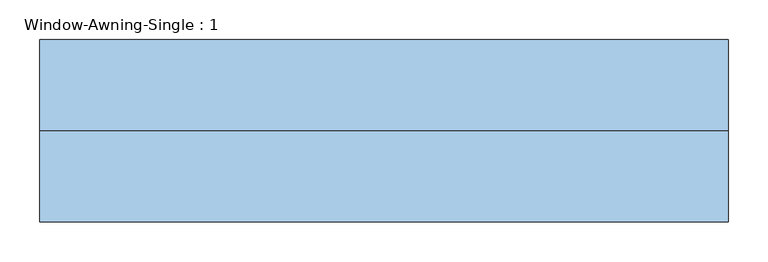
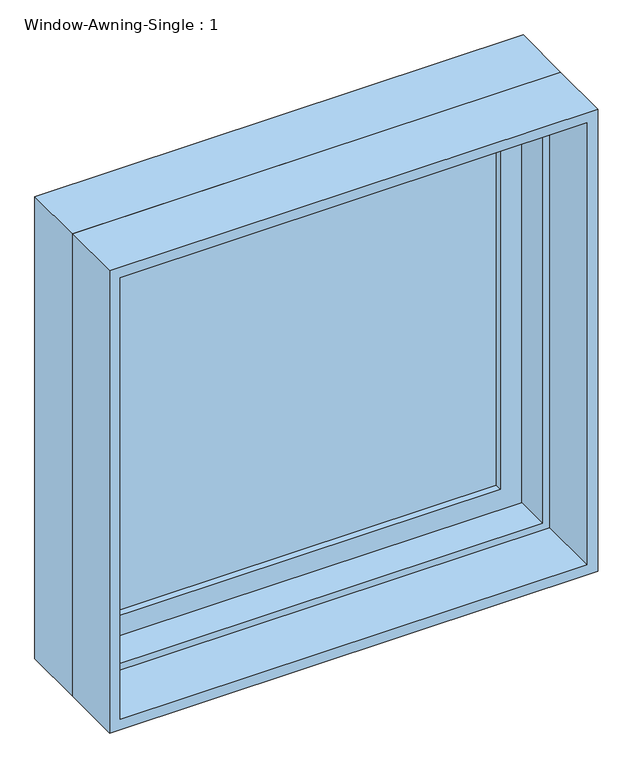
"""IFC4 building model written with IfcOpenShell, lengths in millimetres: window geometry, Window-Awning-Single : 1."""

from ifc_helpers import new_model, si_unit, frame, origin, place, context, project, spatial, polyline, outline, extrude, faceted_brep, source, transform, mapped, element, save


def window_awning_single_1_f21cafb6(model_context):
    return source(origin(), model_context, "Body", "SolidModel", [
        faceted_brep([(419.1, 73.025, 927.1), (419.1, 123.825, 927.1), (-419.1, 123.825, 927.1), (-419.1, 73.025, 927.1), (400.05, 9.525, 946.15), (400.05, 73.025, 946.15), (-400.05, 73.025, 946.15), (-400.05, 9.525, 946.15), (431.8, 123.825, 914.4), (431.8, 9.525, 914.4), (-431.8, 9.525, 914.4), (-431.8, 123.825, 914.4), (-419.1, 123.825, 1765.3), (-419.1, 73.025, 1765.3), (-400.05, 73.025, 1746.25), (-400.05, 9.525, 1746.25), (-431.8, 9.525, 1778.0), (-431.8, 123.825, 1778.0), (419.1, 123.825, 1765.3), (419.1, 73.025, 1765.3), (400.05, 73.025, 1746.25), (400.05, 9.525, 1746.25), (431.8, 9.525, 1778.0), (431.8, 123.825, 1778.0)], [[[0, 1, 2, 3]], [[4, 5, 6, 7]], [[8, 9, 10, 11]], [[3, 2, 12, 13]], [[7, 6, 14, 15]], [[11, 10, 16, 17]], [[13, 12, 18, 19]], [[15, 14, 20, 21]], [[17, 16, 22, 23]], [[11, 17, 23, 8], [1, 18, 12, 2]], [[19, 18, 1, 0]], [[3, 13, 19, 0], [5, 20, 14, 6]], [[21, 20, 5, 4]], [[9, 22, 16, 10], [7, 15, 21, 4]], [[23, 22, 9, 8]]]),
        extrude(outline(polyline([(361.95, 104.775), (361.95, 98.425), (-361.95, 98.425), (-361.95, 104.775), (361.95, 104.775)])), frame((0.0, 0.0, 984.25), z_axis=(0.0, 0.0, 1.0), x_axis=(1.0, 0.0, 0.0)), (0.0, 0.0, 1.0), 723.9),
        extrude(outline(polyline([(361.95, 92.075), (361.95, 85.725), (-361.95, 85.725), (-361.95, 92.075), (361.95, 92.075)])), frame((0.0, 0.0, 984.25), z_axis=(0.0, 0.0, 1.0), x_axis=(1.0, 0.0, 0.0)), (0.0, 0.0, 1.0), 723.9),
        extrude(outline(polyline([(927.1, -419.1), (927.1, 419.1), (1765.3, 419.1), (1765.3, -419.1), (927.1, -419.1)]), holes=[polyline([(1708.15, -361.95), (1708.15, 361.95), (984.25, 361.95), (984.25, -361.95), (1708.15, -361.95)])]), frame((0.0, 73.025, 0.0), z_axis=(0.0, 1.0, 0.0), x_axis=(0.0, 0.0, 1.0)), (0.0, 0.0, 1.0), 44.45),
        extrude(outline(polyline([(1778.0, -431.8), (914.4, -431.8), (914.4, 431.8), (1778.0, 431.8), (1778.0, -431.8)]), holes=[polyline([(1758.95, -412.75), (1758.95, 412.75), (933.45, 412.75), (933.45, -412.75), (1758.95, -412.75)])]), frame((0.0, -104.775, 0.0), z_axis=(0.0, 1.0, 0.0), x_axis=(0.0, 0.0, 1.0)), (0.0, 0.0, 1.0), 114.3),
    ])


if __name__ == "__main__":
    model = new_model("IFC4")
    model_context = context("Model", 3, world=origin())
    ifc_project = project(units=[si_unit("LENGTHUNIT", "METRE", prefix="MILLI")], contexts=[model_context])
    site = spatial("IfcSite", under=ifc_project)
    building = spatial("IfcBuilding", under=site)
    placement = place(None, origin())
    window_awning_single_1_shape = window_awning_single_1_f21cafb6(model_context)
    element("IfcWindow", 1, ObjectType="Window-Awning-Single : 1", at=placement, inside=building, context=model_context, shape_type="MappedRepresentation", body=[
        mapped(window_awning_single_1_shape, transform((0.0, 0.0, 0.0), x_axis=(1.0, 0.0, 0.0), y_axis=(0.0, 1.0, 0.0), z_axis=(0.0, 0.0, 1.0))),
    ])
    save(model, "model.ifc")

# Revit data of these elements
# Type "Window-Awning-Single : 1"
#   Type Mark = "14"
#   Fire Rating = "0.5h"
#   Assembly Code = "B2020100"
#   Analytic Construction = "Double glazing - domestic"
#   Window Inset [instance default] = 0' - 0"
#   Wall Thickness [instance default] = 0' - 6"
#   Visual Light Transmittance = 0.81
#   Thermal Resistance (R) = 0.319569 (m²·K)/W
#   Solar Heat Gain Coefficient = 0.76
#   Rough Width = 2' - 10 1/2"
#   Rough Height = 2' - 10 1/2"
#   Interior Wall Closure [instance default] = 0' - 2 1/4"
#   Height = 2' - 10"
#   Heat Transfer Coefficient (U) = 3.12929 W/(m²·K)
#   Frame Extension [instance default] = 0' - 0 1/4"
#   Exterior Wall Closure [instance default] = 0' - 1 1/4"
#   Extension Jamb [instance default] = 0' - 2 1/4"
#   Default Sill Height = 3' - 0"
#   Width = 2' - 10"
#   Muntin Visibility = yes
#   Interior Trim Visibility [instance default] = yes
#   Exterior Trim Visibility [instance default] = yes
#   Extension Jamb Visibility [instance default] = yes
#   Muntin Pattern = Muntin Pattern_2x2 : Muntin Pattern_2x2
#   Interior Trim Material = 1X WOOD COMPOSITE TRIM
#   Interior Trim = Trim-Window-Interior-Flat : Picture Frame
#   Interior Frame Material = 1X WOOD COMPOSITE TRIM
#   Glass Panel Material = NEW DOUBLE HUNG WINDOWS (TYP.)
#   Exterior Trim Material = 1X WOOD COMPOSITE TRIM
#   Exterior Trim = Trim-Window-Exterior-Flat : with Sill
#   Exterior Frame Material = 1X WOOD COMPOSITE TRIM
#   Wall Closure = (empty or 0)
# Element 1 (IfcWindow, "Window-Awning-Single : 1")
#   Wall Thickness = 0' - 8 1/4"
#   Extension Jamb = 0' - 4 1/2"
#   Materials on its faces: "1X WOOD COMPOSITE TRIM", "NEW DOUBLE HUNG WINDOWS (TYP.)", "Clad - White"
# Materials
#   "1X WOOD COMPOSITE TRIM": class "Generic", colour RGB 88 61 61, transparency 0, Cost = 0
#   "NEW DOUBLE HUNG WINDOWS (TYP.)": class "Glass", colour RGB 218 227 224, transparency 0.85, Description = "Soda Lime Glass", Cost = 0
#   "Clad - White": class "Wood", colour RGB 242 242 238, transparency 0, Cost = 0
